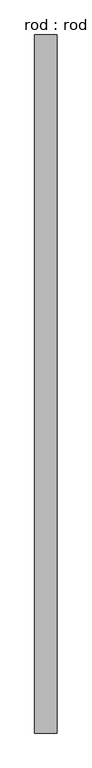
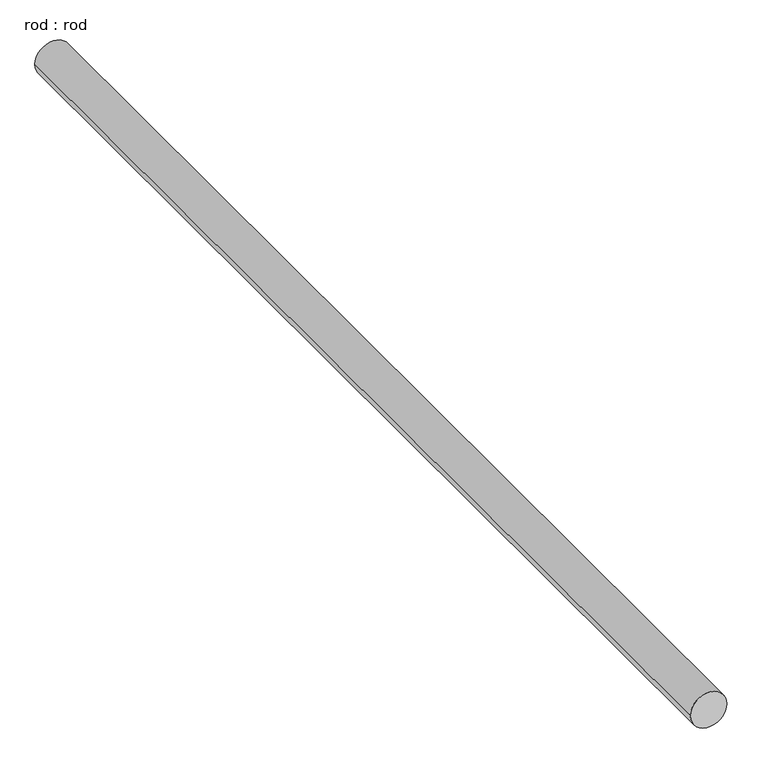
"""IFC4 building model written with IfcOpenShell, lengths in millimetres: proxy geometry, rod : rod."""

from ifc_helpers import new_model, si_unit, point, frame, frame_2d, origin, place, context, project, spatial, circle_curve, trimmed, segment, composite_curve, outline, extrude, source, transform, mapped, element, save


def rod_rod_e4310c48(model_context):
    return source(origin(), model_context, "Body", "SweptSolid", [
        extrude(outline(composite_curve([segment(trimmed(circle_curve(frame_2d((0.0108462, 0.0)), 200.0), [point((0.0108462, 200.0))], [point((0.0108462, -200.0))], False, "CARTESIAN"), True, "CONTINUOUS"), segment(trimmed(circle_curve(frame_2d((0.0108462, 0.0)), 200.0), [point((0.0108462, -200.0))], [point((0.0108462, 200.0))], False, "CARTESIAN"), True, "CONTINUOUS")], self_intersect=False)), frame((0.0, -2121.0466531, 0.0), z_axis=(0.0, 1.0, 0.0), x_axis=(0.0, 0.0, 1.0)), (0.0, 0.0, 1.0), 12427.5505368),
    ])


if __name__ == "__main__":
    model = new_model("IFC4")
    model_context = context("Model", 3, world=origin())
    ifc_project = project(units=[si_unit("LENGTHUNIT", "METRE", prefix="MILLI")], contexts=[model_context])
    site = spatial("IfcSite", under=ifc_project)
    building = spatial("IfcBuilding", under=site)
    placement = place(None, origin())
    rod_rod_shape = rod_rod_e4310c48(model_context)
    element("IfcBuildingElementProxy", 1, Name="rod : rod", ObjectType="rod : rod", at=placement, inside=building, context=model_context, shape_type="MappedRepresentation", body=[
        mapped(rod_rod_shape, transform((0.0, 0.0, 0.0), x_axis=(1.0, 0.0, 0.0), y_axis=(0.0, 1.0, 0.0), z_axis=(0.0, 0.0, 1.0))),
    ])
    save(model, "model.ifc")

# Revit data of these elements
# Type "rod : rod"
#   Default Elevation = 0
